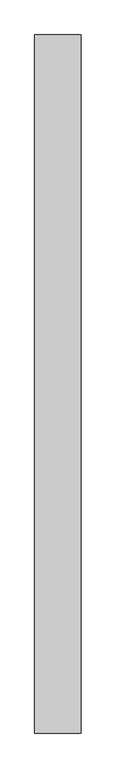
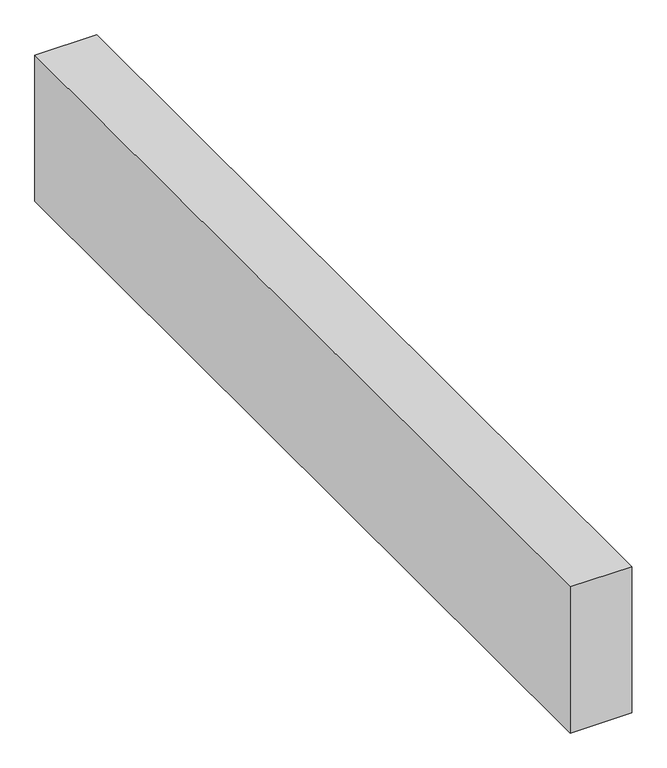
"""IFC4 building model written with IfcOpenShell, lengths in millimetres: proxy geometry, Space Planning Box_hec : Space Planning Box_hec."""

import ifcopenshell
import ifcopenshell.guid

model = None  # the IFC model being written
_history = None  # IfcOwnerHistory: only IFC2X3 demands one
_inside = {}  # id of a spatial element -> (the spatial element, [elements in it])
_under = {}  # id of a project, library or spatial element -> (it, [spatial elements below it])
_declared = {}  # id of a project -> (the project, [libraries it declares])
_typed = {}  # id of a type object -> (the type object, [elements of that type])
_made_of = {}  # id of a material, layer set ... -> (it, [elements and type objects made of it])


def new_model(schema):
    """Start an empty IFC model of exactly this schema.

    Asked for "IFC4X3", IfcOpenShell would pick the latest addendum, in which some entities
    have other attributes; the version numbers below select the first issue.
    IFC2X3 requires an IfcOwnerHistory on every rooted entity: one is made here for all.
    """
    global model, _history
    if schema == "IFC4X3":
        model = ifcopenshell.file(schema_version=(4, 3, 0, 0))
    else:
        model = ifcopenshell.file(schema=schema)
    _inside.clear()
    _under.clear()
    _declared.clear()
    _typed.clear()
    _made_of.clear()
    _history = None
    if model.schema == "IFC2X3":
        org = make("IfcOrganization", Name="unknown")
        user = make(
            "IfcPersonAndOrganization",
            ThePerson=make("IfcPerson", FamilyName="unknown"),
            TheOrganization=org,
        )
        app = make(
            "IfcApplication",
            ApplicationDeveloper=org,
            Version="unknown",
            ApplicationFullName="unknown",
            ApplicationIdentifier="unknown",
        )
        _history = make(
            "IfcOwnerHistory",
            OwningUser=user,
            OwningApplication=app,
            ChangeAction="ADDED",
            CreationDate=0,
        )
    return model


def make(cls, **values):
    """One entity of the class cls with the attributes given. An attribute that is None is left unset."""
    return model.create_entity(
        cls, **{name: value for name, value in values.items() if value is not None}
    )


def rooted(cls, **values):
    """An entity with a GlobalId (a new one), such as an element, a storey or a relation."""
    return make(cls, GlobalId=ifcopenshell.guid.new(), OwnerHistory=_history, **values)


def si_unit(unit_type, name, prefix=None):
    """IfcSIUnit, for example si_unit("LENGTHUNIT", "METRE", prefix="MILLI")."""
    return make("IfcSIUnit", UnitType=unit_type, Prefix=prefix, Name=name)


def assignment(units):
    """IfcUnitAssignment: the units of a project."""
    return None if units is None else make("IfcUnitAssignment", Units=units)


def point(xyz):
    """IfcCartesianPoint."""
    return None if xyz is None else make("IfcCartesianPoint", Coordinates=xyz)


def direction(xyz):
    """IfcDirection."""
    return None if xyz is None else make("IfcDirection", DirectionRatios=xyz)


def frame(location, z_axis=None, x_axis=None):
    """IfcAxis2Placement3D, a coordinate frame: its origin and axes. An axis left out is left unset."""
    return make(
        "IfcAxis2Placement3D",
        Location=point(location),
        Axis=direction(z_axis),
        RefDirection=direction(x_axis),
    )


def origin():
    """The frame at (0, 0, 0) with its axes left unset."""
    return frame((0.0, 0.0, 0.0))


def origin_with_axes():
    """The frame at (0, 0, 0) with the z axis (0, 0, 1) and the x axis (1, 0, 0) written out."""
    return frame((0.0, 0.0, 0.0), z_axis=(0.0, 0.0, 1.0), x_axis=(1.0, 0.0, 0.0))


def place(relative_to, where):
    """IfcLocalPlacement: puts the frame where relative to a parent placement (None: the world)."""
    return make(
        "IfcLocalPlacement", PlacementRelTo=relative_to, RelativePlacement=where
    )


def context(
    kind, dimensions, precision=None, world=None, true_north=None, identifier=None
):
    """IfcGeometricRepresentationContext, for example the 3D "Model" context."""
    return make(
        "IfcGeometricRepresentationContext",
        ContextIdentifier=identifier,
        ContextType=kind,
        CoordinateSpaceDimension=dimensions,
        Precision=precision,
        WorldCoordinateSystem=world,
        TrueNorth=true_north,
    )


def project(units=None, contexts=None):
    """IfcProject with its units and contexts."""
    return rooted(
        "IfcProject",
        Name="project",
        RepresentationContexts=contexts,
        UnitsInContext=assignment(units),
    )


def spatial(cls, under=None, at=None, **own):
    """A site, building, storey or space (cls), placed at a placement, below another one or the project."""
    s = rooted(cls, ObjectPlacement=at, **own)
    if under is not None:
        _under.setdefault(under.id(), (under, []))[1].append(s)
    return s


def polyline(points):
    """IfcPolyline through the points."""
    return make("IfcPolyline", Points=[point(p) for p in points])


def outline(outer, holes=None, kind="AREA"):
    """IfcArbitraryClosedProfileDef: a profile drawn as a closed curve; with holes, ...WithVoids."""
    if holes is None:
        return make("IfcArbitraryClosedProfileDef", ProfileType=kind, OuterCurve=outer)
    return make(
        "IfcArbitraryProfileDefWithVoids",
        ProfileType=kind,
        OuterCurve=outer,
        InnerCurves=holes,
    )


def extrude(swept, where, along, depth):
    """IfcExtrudedAreaSolid: the profile swept, set in the frame where, extruded along a direction by depth."""
    return make(
        "IfcExtrudedAreaSolid",
        SweptArea=swept,
        Position=where,
        ExtrudedDirection=direction(along),
        Depth=depth,
    )


def shape(context_of_items, identifier, shape_type, items):
    """IfcShapeRepresentation: the items that make up one representation, for example the "Body"."""
    return make(
        "IfcShapeRepresentation",
        ContextOfItems=context_of_items,
        RepresentationIdentifier=identifier,
        RepresentationType=shape_type,
        Items=items,
    )


def source(mapping_origin, context_of_items, identifier, shape_type, items):
    """IfcRepresentationMap: a shape defined once, which mapped items show again and again."""
    return make(
        "IfcRepresentationMap",
        MappingOrigin=mapping_origin,
        MappedRepresentation=shape(context_of_items, identifier, shape_type, items),
    )


def transform(
    local_origin,
    x_axis=None,
    y_axis=None,
    z_axis=None,
    scale=None,
    scale2=None,
    scale3=None,
    uniform=True,
):
    """IfcCartesianTransformationOperator3D, or its non-uniform kind. x_axis, y_axis, z_axis: its Axis1, 2, 3."""
    if uniform:
        return make(
            "IfcCartesianTransformationOperator3D",
            Axis1=direction(x_axis),
            Axis2=direction(y_axis),
            LocalOrigin=point(local_origin),
            Scale=scale,
            Axis3=direction(z_axis),
        )
    return make(
        "IfcCartesianTransformationOperator3DnonUniform",
        Axis1=direction(x_axis),
        Axis2=direction(y_axis),
        LocalOrigin=point(local_origin),
        Scale=scale,
        Axis3=direction(z_axis),
        Scale2=scale2,
        Scale3=scale3,
    )


def mapped(mapping_source, mapping_target):
    """IfcMappedItem: shows the shape of a source again, moved by a transform."""
    return make(
        "IfcMappedItem", MappingSource=mapping_source, MappingTarget=mapping_target
    )


def made_of(thing, what):
    """Note that an element or type object is made of a material, layer set ...; save() writes the relation."""
    if what is not None:
        _made_of.setdefault(what.id(), (what, []))[1].append(thing)
    return thing


def element(
    cls,
    number,
    at=None,
    inside=None,
    cuts=None,
    type_object=None,
    material=None,
    context=None,
    identifier="Body",
    shape_type=None,
    held_by="IfcProductDefinitionShape",
    body=None,
    shapes=None,
    **own,
):
    """One element of the class cls, such as IfcWall. Its Tag is "e" and its number.

    at: its placement. inside: the storey or other place that contains it. cuts: it is an
    opening in that element (IfcRelVoidsElement). A single representation is given by context,
    identifier, shape_type and body (its items); several are given by shapes. held_by: the class
    of the entity that holds the representations. save() writes the other relations.
    """
    e = rooted(cls, Tag="e%d" % number, ObjectPlacement=at, **own)
    if body is not None:
        shapes = [shape(context, identifier, shape_type, body)]
    if shapes is not None:
        e.Representation = make(held_by, Representations=shapes)
    if inside is not None:
        _inside.setdefault(inside.id(), (inside, []))[1].append(e)
    if cuts is not None:
        rooted(
            "IfcRelVoidsElement", RelatingBuildingElement=cuts, RelatedOpeningElement=e
        )
    if type_object is not None:
        _typed.setdefault(type_object.id(), (type_object, []))[1].append(e)
    return made_of(e, material)


def aggregate(whole, parts):
    """IfcRelAggregates: a whole, such as a stair, and the parts it consists of."""
    return rooted("IfcRelAggregates", RelatingObject=whole, RelatedObjects=parts)


def save(model, path):
    """Write the relations noted so far, then the file.

    IfcRelAggregates (storeys below a building ...), IfcRelContainedInSpatialStructure (elements
    in a storey), IfcRelDefinesByType, IfcRelAssociatesMaterial and IfcRelDeclares: one each for
    every whole, place, type object, material and project.
    """
    for whole, parts in _under.values():
        aggregate(whole, parts)
    for where, things in _inside.values():
        rooted(
            "IfcRelContainedInSpatialStructure",
            RelatedElements=things,
            RelatingStructure=where,
        )
    for kind, things in _typed.values():
        rooted("IfcRelDefinesByType", RelatedObjects=things, RelatingType=kind)
    for what, things in _made_of.values():
        rooted("IfcRelAssociatesMaterial", RelatedObjects=things, RelatingMaterial=what)
    for by, libraries in _declared.values():
        rooted("IfcRelDeclares", RelatingContext=by, RelatedDefinitions=libraries)
    model.write(path)


def generic_models_03d31222(model_context):
    return source(origin(), model_context, "Body", "SweptSolid", [
        extrude(outline(polyline([(1200.0, 18000.0), (1200.0, -18000.0), (-1200.0, -18000.0), (-1200.0, 18000.0), (1200.0, 18000.0)])), origin_with_axes(), (0.0, 0.0, 1.0), 6000.0),
    ])


if __name__ == "__main__":
    model = new_model("IFC4")
    model_context = context("Model", 3, world=origin())
    ifc_project = project(units=[si_unit("LENGTHUNIT", "METRE", prefix="MILLI")], contexts=[model_context])
    site = spatial("IfcSite", under=ifc_project)
    building = spatial("IfcBuilding", under=site)
    placement = place(None, origin())
    generic_models_shape = generic_models_03d31222(model_context)
    element("IfcBuildingElementProxy", 1, Name="Space Planning Box_hec : Space Planning Box_hec", ObjectType="Space Planning Box_hec : Space Planning Box_hec", at=placement, inside=building, context=model_context, shape_type="MappedRepresentation", body=[
        mapped(generic_models_shape, transform((0.0, 0.0, 0.0), x_axis=(1.0, 0.0, 0.0), y_axis=(0.0, 1.0, 0.0), z_axis=(0.0, 0.0, 1.0))),
    ])
    save(model, "model.ifc")

# Revit data of these elements
# Type "Space Planning Box_hec : Space Planning Box_hec"
#   Type Comments = "..."
#   Room Name [instance default] = "?"
#   Interior Finish [instance default] = ""
#   Exterior Finish [instance default] = ""
#   Department [instance default] = ""
#   Assembly Code = "..."
#   Width [instance default] = 1524 mm
#   Program Area [instance default] = 0.00 m²
#   Length [instance default] = 1524 mm
#   Height [instance default] = 1524 mm
#   Area [instance default] = 2.32258 m²
#   Fill Color [instance default] = Cyan
#   Default Elevation = 0
# Element 1 (IfcBuildingElementProxy, "Space Planning Box_hec : Space Planning Box_hec")
#   Room Name = "Corridor"
#   Interior Finish = "IF2-1"
#   Exterior Finish = "EF1"
#   Department = "AR"
#   Width = 2400 mm
#   Program Area = 86.40 m²
#   Length = 36000 mm
#   Height = 6000 mm
#   Area = 86.40 m²
#   Fill Color = Lavender
#   Materials on its faces: "Lavender"
# Materials
#   "Cyan": class "Generic", colour RGB 0 255 255, transparency 0.2, Cost = 0
#   "Lavender": class "Generic", colour RGB 186 85 211, transparency 0.2, Cost = 0
